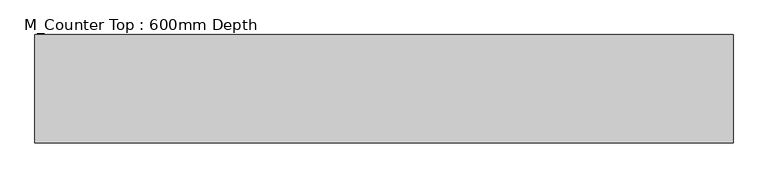
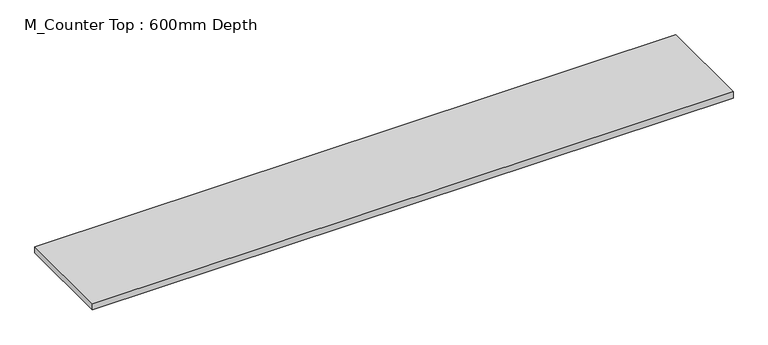
"""IFC4 building model written with IfcOpenShell, lengths in millimetres: furniture geometry, M_Counter Top : 600mm Depth."""

from ifc_helpers import new_model, si_unit, frame, origin, place, context, project, spatial, polyline, outline, extrude, source, transform, mapped, element, save


def m_counter_top_600mm_depth_a21ada81(model_context):
    return source(origin(), model_context, "Body", "SweptSolid", [
        extrude(outline(polyline([(2823.5377049, 0.0), (2823.5377049, -625.0), (-1200.4622951, -625.0), (-1200.4622951, 0.0), (2823.5377049, 0.0)])), frame((0.0, 0.0, 860.0), z_axis=(0.0, 0.0, 1.0), x_axis=(1.0, 0.0, 0.0)), (0.0, 0.0, 1.0), 40.0),
    ])


if __name__ == "__main__":
    model = new_model("IFC4")
    model_context = context("Model", 3, world=origin())
    ifc_project = project(units=[si_unit("LENGTHUNIT", "METRE", prefix="MILLI")], contexts=[model_context])
    site = spatial("IfcSite", under=ifc_project)
    building = spatial("IfcBuilding", under=site)
    placement = place(None, origin())
    m_counter_top_600mm_depth_shape = m_counter_top_600mm_depth_a21ada81(model_context)
    element("IfcFurniture", 1, ObjectType="M_Counter Top : 600mm Depth", at=placement, inside=building, context=model_context, shape_type="MappedRepresentation", body=[
        mapped(m_counter_top_600mm_depth_shape, transform((0.0, 0.0, 0.0), x_axis=(1.0, 0.0, 0.0), y_axis=(0.0, 1.0, 0.0), z_axis=(0.0, 0.0, 1.0))),
    ])
    save(model, "model.ifc")

# Revit data of these elements
# Type "M_Counter Top : 600mm Depth"
#   AccessibilityPerformance = "AccessibilityPerformance"
#   CodePerformance = "CodePerformance"
#   Area = "Area"
#   Color = "Color"
#   Constituents = "Constituents"
#   Features = "Features"
#   Finish = "Finish"
#   Grade = "Grade"
#   Material = "Material"
#   ModelReference = "ModelReference"
#   NominalHeight = "NominalHeight"
#   NominalLength = "NominalLength"
#   NominalWidth = "NominalWidth"
#   ProductionYear = "ProductionYear"
#   Reference = "Reference"
#   Shape = "Shape"
#   Size = "Size"
#   SustainabilityPerformance = "SustainabilityPerformance"
#   WarrantyDescription = "WarrantyDescription"
#   WarrantyDurationLabor = "WarrantyDurationLabor"
#   WarrantyDurationParts = "WarrantyDurationParts"
#   WarrantyGuarantorLabor = "WarrantyGuarantorLabor"
#   WarrantyGuarantorParts = "WarrantyGuarantorParts"
#   ExpectedLife = "ExpectedLife"
#   ReplacementCost = "ReplacementCost"
#   AssetAccountingType = "FIXED"
#   ModelLabel = "ModelLabel"
#   Manufacturer = "Manufacturer"
#   Finish = "Finish"
#   Construction Type = "Construction Type"
#   Counter Thickness = 0.040 m
#   Depth = 0.625 m
#   Height = 0.900 m
#   Length [instance default] = 2.500 m
#   Backsplash Visibility [instance default] = yes
#   Counter Top Material = none
#   Assembly Code = ""
# Element 1 (IfcFurniture, "M_Counter Top : 600mm Depth")
#   Length = 4.024 m
#   Backsplash Visibility = no
#   Materials on its faces: "Counter Top"
# Materials
#   "Counter Top": class "Wood", colour RGB 226 177 128, transparency 0
